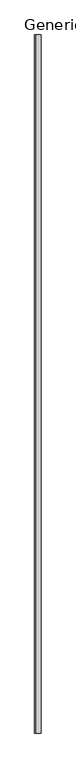
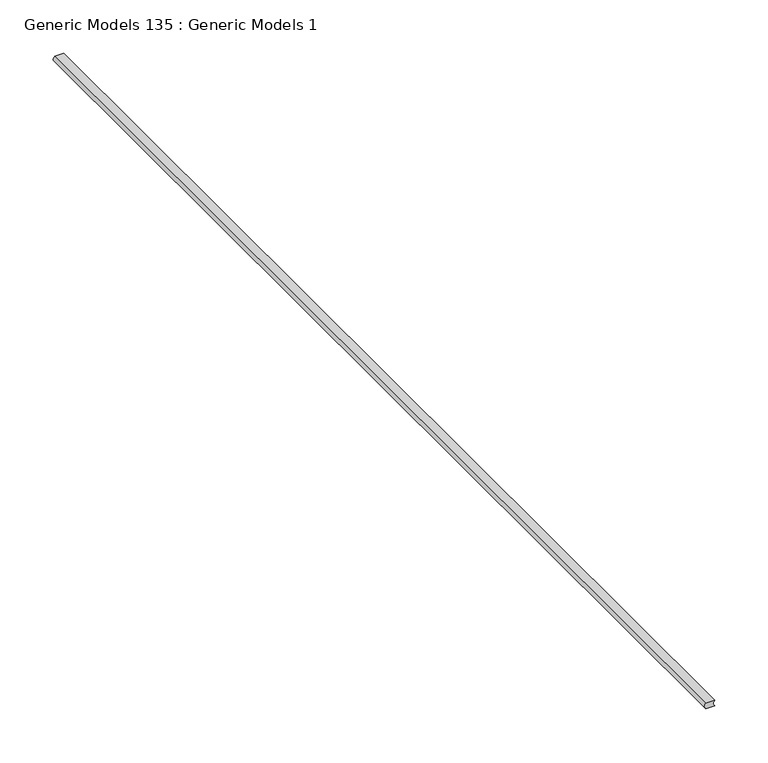
"""IFC4 building model written with IfcOpenShell, lengths in millimetres: proxy geometry, Generic Models 135 : Generic Models 1."""

from ifc_helpers import new_model, si_unit, point, frame, frame_2d, origin, place, context, project, spatial, polyline, circle_curve, trimmed, segment, composite_curve, outline, extrude, source, transform, mapped, element, save


def generic_models_135_generic_models_1_f6c730d4(model_context):
    return source(origin(), model_context, "Body", "SweptSolid", [
        extrude(outline(composite_curve([segment(trimmed(circle_curve(frame_2d((-2147.2483876, 51035.5452774)), 4.3100275), [point((-2150.4233876, 51032.6305369))], [point((-2144.0733876, 51032.6305369))], True, "CARTESIAN"), True, "CONTINUOUS"), segment(polyline([(-2144.0733876, 51032.6305369), (-2144.0733876, 51023.1055369)]), True, "CONTINUOUS"), segment(trimmed(circle_curve(frame_2d((-2147.2483876, 51026.0202774)), 4.3100275), [point((-2144.0733876, 51023.1055369))], [point((-2150.4233876, 51023.1055369))], False, "CARTESIAN"), True, "CONTINUOUS"), segment(polyline([(-2150.4233876, 51023.1055369), (-2150.4233876, 51032.6305369)]), True, "CONTINUOUS")], self_intersect=False)), frame((0.0, 0.0, 0.0), z_axis=(0.0, 1.0, 0.0), x_axis=(0.0, 0.0, 1.0)), (0.0, 0.0, 1.0), 1219.2),
    ])


if __name__ == "__main__":
    model = new_model("IFC4")
    model_context = context("Model", 3, world=origin())
    ifc_project = project(units=[si_unit("LENGTHUNIT", "METRE", prefix="MILLI")], contexts=[model_context])
    site = spatial("IfcSite", under=ifc_project)
    building = spatial("IfcBuilding", under=site)
    placement = place(None, origin())
    generic_models_135_generic_models_1_shape = generic_models_135_generic_models_1_f6c730d4(model_context)
    element("IfcBuildingElementProxy", 1, Name="Generic Models 135 : Generic Models 1", ObjectType="Generic Models 135 : Generic Models 1", at=placement, inside=building, context=model_context, shape_type="MappedRepresentation", body=[
        mapped(generic_models_135_generic_models_1_shape, transform((0.0, 0.0, 0.0), x_axis=(1.0, 0.0, 0.0), y_axis=(0.0, 1.0, 0.0), z_axis=(0.0, 0.0, 1.0))),
    ])
    save(model, "model.ifc")

# Revit data of these elements
# Element 1 (IfcBuildingElementProxy, "Generic Models 135 : Generic Models 1")
#   Materials on its faces: "SEALANT (W/ BACKER ROD IF NECESSARY)"
# Materials
#   "SEALANT (W/ BACKER ROD IF NECESSARY)": class "Unassigned", colour RGB 120 120 120, transparency 0, Cost = 0
